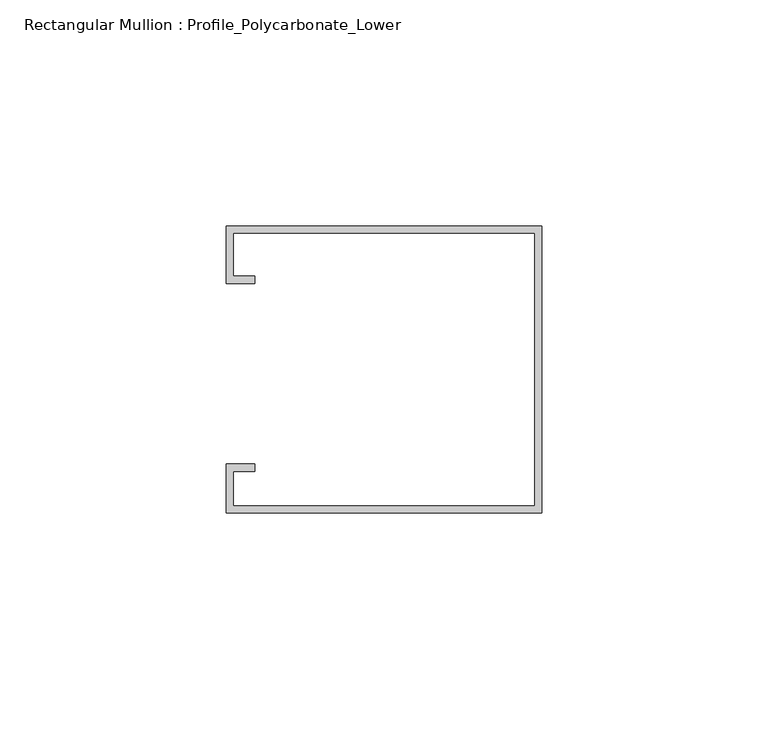
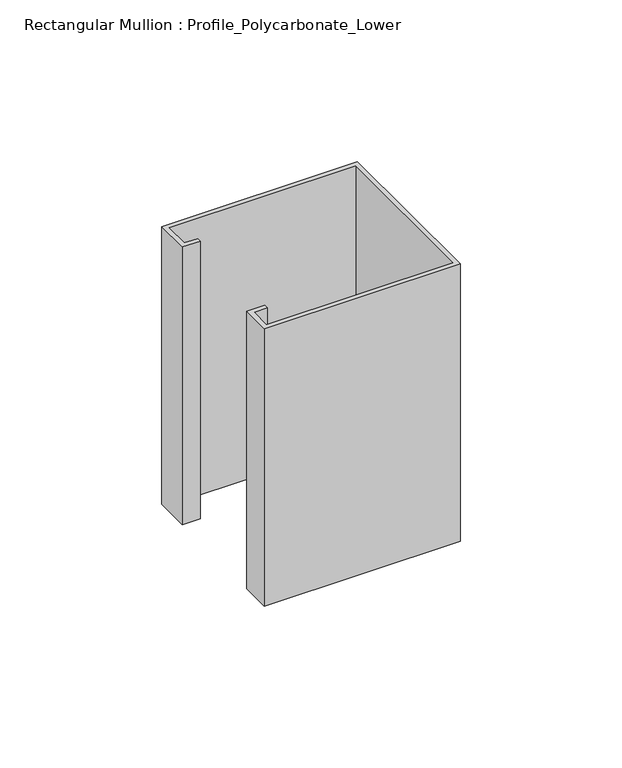
"""IFC4 building model written with IfcOpenShell, lengths in millimetres: member geometry, Rectangular Mullion : Profile_Polycarbonate_Lower."""

from ifc_helpers import new_model, si_unit, frame, origin, place, context, project, spatial, polyline, outline, extrude, source, transform, mapped, element, save


def rectangular_mullion_profile_polycarbonate_lower_5c02ef7d(model_context):
    return source(origin(), model_context, "Body", "SweptSolid", [
        extrude(outline(polyline([(0.0, 32.7), (0.0, -30.8), (-69.85, -30.8), (-69.85, -20.0), (-63.5, -20.0), (-63.5, -21.5875), (-68.2625, -21.5875), (-68.2625, -29.2125), (-1.5875, -29.2125), (-1.5875, 31.1125), (-68.2625, 31.1125), (-68.2625, 21.5875), (-63.5, 21.5875), (-63.5, 20.0), (-69.85, 20.0), (-69.85, 32.7), (0.0, 32.7)])), frame((0.0, 0.0, -104.775), z_axis=(0.0, 0.0, 1.0), x_axis=(1.0, 0.0, 0.0)), (0.0, 0.0, 1.0), 104.775),
    ])


if __name__ == "__main__":
    model = new_model("IFC4")
    model_context = context("Model", 3, world=origin())
    ifc_project = project(units=[si_unit("LENGTHUNIT", "METRE", prefix="MILLI")], contexts=[model_context])
    site = spatial("IfcSite", under=ifc_project)
    building = spatial("IfcBuilding", under=site)
    placement = place(None, origin())
    rectangular_mullion_profile_polycarbonate_lower_shape = rectangular_mullion_profile_polycarbonate_lower_5c02ef7d(model_context)
    element("IfcMember", 1, ObjectType="Rectangular Mullion : Profile_Polycarbonate_Lower", at=placement, inside=building, context=model_context, shape_type="MappedRepresentation", body=[
        mapped(rectangular_mullion_profile_polycarbonate_lower_shape, transform((0.0, 0.0, 0.0), x_axis=(1.0, 0.0, 0.0), y_axis=(0.0, 1.0, 0.0), z_axis=(0.0, 0.0, 1.0))),
    ])
    save(model, "model.ifc")

# Revit data of these elements
# Type "Rectangular Mullion : Profile_Polycarbonate_Lower"
#   built-in parameter 1007322 = 0.208333 (stored number, unit not read)
#   built-in parameter 1007321 = 0 (stored number, unit not read)
#   built-in parameter 1007320 = 0.00520833 (stored number, unit not read)
# Element 1 (IfcMember, "Rectangular Mullion : Profile_Polycarbonate_Lower")
#   Materials on its faces: "GALVANIZED UNISTRUT P5500, 1 5/8\" X 2 7/16\" OR ALUM. CHANNEL"
# Materials
#   "GALVANIZED UNISTRUT P5500, 1 5/8\" X 2 7/16\" OR ALUM. CHANNEL": class "Metal", colour RGB 244 244 244, transparency 0, Description = "Aluminum 6061", Cost = 0
